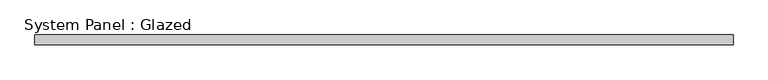
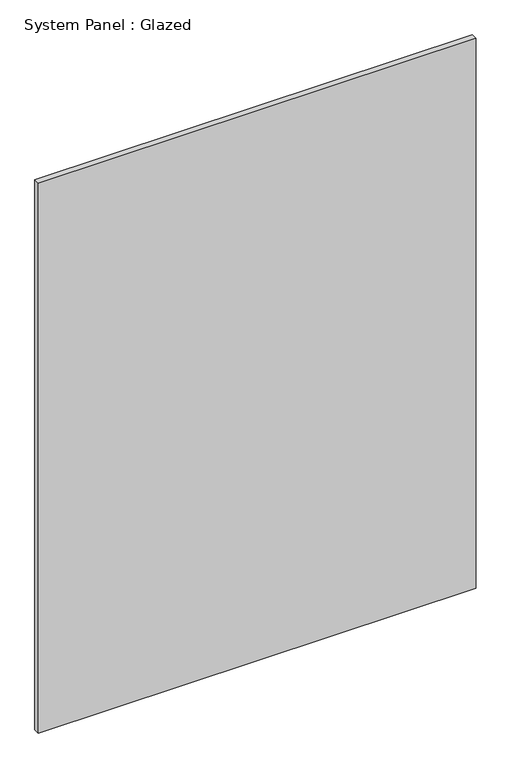
"""IFC4 building model written with IfcOpenShell, lengths in millimetres: plate geometry, System Panel : Glazed."""

from ifc_helpers import new_model, si_unit, origin, origin_with_axes, place, context, project, spatial, polyline, outline, extrude, source, transform, mapped, element, save


def system_panel_glazed_1c65ff95(model_context):
    return source(origin(), model_context, "Body", "SweptSolid", [
        extrude(outline(polyline([(902.5000002, 24.5), (-902.5000002, 24.5), (-902.5000002, 49.5), (902.5000002, 49.5), (902.5000002, 24.5)])), origin_with_axes(), (0.0, 0.0, 1.0), 2395.0),
    ])


if __name__ == "__main__":
    model = new_model("IFC4")
    model_context = context("Model", 3, world=origin())
    ifc_project = project(units=[si_unit("LENGTHUNIT", "METRE", prefix="MILLI")], contexts=[model_context])
    site = spatial("IfcSite", under=ifc_project)
    building = spatial("IfcBuilding", under=site)
    placement = place(None, origin())
    system_panel_glazed_shape = system_panel_glazed_1c65ff95(model_context)
    element("IfcPlate", 1, ObjectType="System Panel : Glazed", at=placement, inside=building, context=model_context, shape_type="MappedRepresentation", body=[
        mapped(system_panel_glazed_shape, transform((0.0, 0.0, 0.0), x_axis=(1.0, 0.0, 0.0), y_axis=(0.0, 1.0, 0.0), z_axis=(0.0, 0.0, 1.0))),
    ])
    save(model, "model.ifc")

# Revit data of these elements
# Element 1 (IfcPlate, "System Panel : Glazed")
#   Materials on its faces: "Glass"
# Materials
#   "Glass": class "Glass", colour RGB 218 227 224, transparency 0.85, Description = "Soda Lime Glass", Cost = 0
